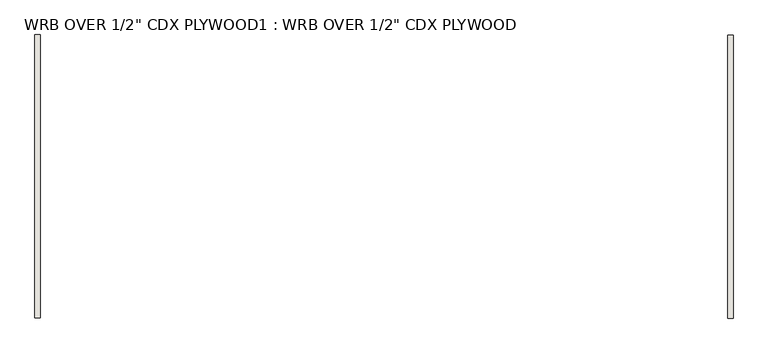
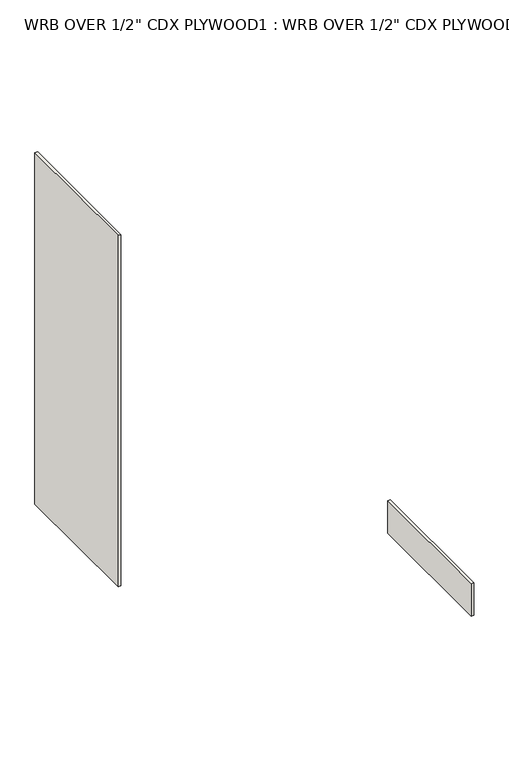
"""IFC4 building model written with IfcOpenShell, lengths in millimetres: wall geometry."""

from ifc_helpers import new_model, si_unit, frame, origin, place, context, project, spatial, polyline, outline, extrude, source, transform, mapped, element, save


def wall_e0b61662(model_context):
    return source(origin(), model_context, "Body", "SweptSolid", [
        extrude(outline(polyline([(24968.9870052, -2319.6634634), (24956.2870052, -2319.6634634), (24956.2870052, -1633.8634634), (24968.9870052, -1633.8634634), (24968.9870052, -2319.6634634)])), frame((0.0, 0.0, 2197.1), z_axis=(0.0, 0.0, 1.0), x_axis=(1.0, 0.0, 0.0)), (0.0, 0.0, 1.0), 164.2249455),
        extrude(outline(polyline([(23292.5870052, -2319.6634634), (23279.8870052, -2319.6634634), (23279.8870052, -1633.8634634), (23292.5870052, -1633.8634634), (23292.5870052, -2319.6634634)])), frame((0.0, 0.0, 2931.649464), z_axis=(0.0, 0.0, 1.0), x_axis=(1.0, 0.0, 0.0)), (0.0, 0.0, 1.0), 1764.62465),
    ])


if __name__ == "__main__":
    model = new_model("IFC4")
    model_context = context("Model", 3, world=origin())
    ifc_project = project(units=[si_unit("LENGTHUNIT", "METRE", prefix="MILLI")], contexts=[model_context])
    site = spatial("IfcSite", under=ifc_project)
    building = spatial("IfcBuilding", under=site)
    placement = place(None, origin())
    wall_shape = wall_e0b61662(model_context)
    element("IfcWall", 1, ObjectType="WRB OVER 1/2\" CDX PLYWOOD1 : WRB OVER 1/2\" CDX PLYWOOD", at=placement, inside=building, context=model_context, shape_type="MappedRepresentation", body=[
        mapped(wall_shape, transform((0.0, 0.0, 0.0), x_axis=(1.0, 0.0, 0.0), y_axis=(0.0, 1.0, 0.0), z_axis=(0.0, 0.0, 1.0))),
    ])
    save(model, "model.ifc")

# Revit data of these elements
# Element 1 (IfcWall, "WRB OVER 1/2\" CDX PLYWOOD1 : WRB OVER 1/2\" CDX PLYWOOD")
#   Materials on its faces: "WRB OVER 1\" STRUCTURAL INSULATED SHEATHING (R-3.6)", "1/2\" CDX PLYWOOD"
# Materials
#   "WRB OVER 1\" STRUCTURAL INSULATED SHEATHING (R-3.6)": class "Unassigned", colour RGB 196 177 123, transparency 0, Cost = 0
#   "1/2\" CDX PLYWOOD": class "Unassigned", colour RGB 196 177 123, transparency 0, Cost = 0
